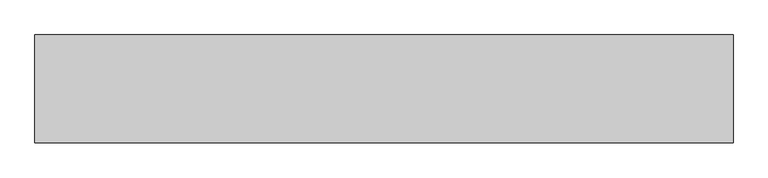
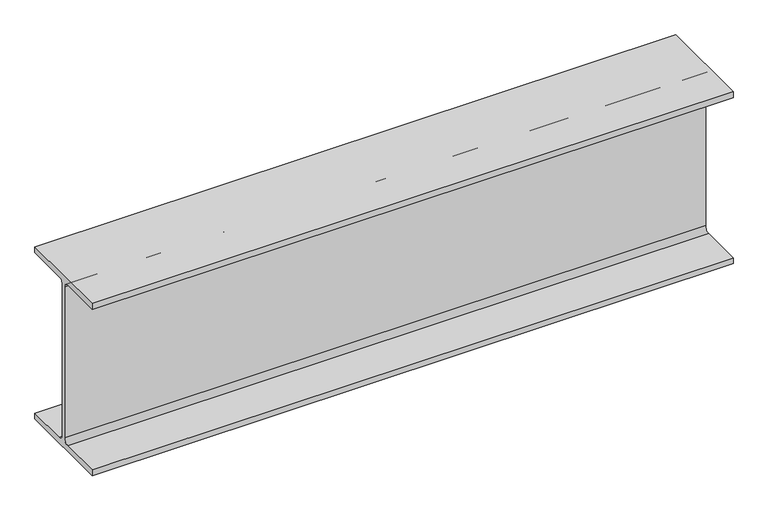
"""IFC4 building model written with IfcOpenShell, lengths in millimetres: beam geometry, Steel Beam_H-KSD3502 : H_SB_ASB_H-194x150x6x9."""

from ifc_helpers import new_model, si_unit, point, frame, frame_2d, origin, place, context, project, spatial, polyline, circle_curve, trimmed, segment, composite_curve, outline, extrude, source, transform, mapped, element, save


def beam_dbf2e1a8(model_context):
    return source(origin(), model_context, "Body", "SweptSolid", [
        extrude(outline(composite_curve([segment(polyline([(-82.5, -141.5), (-11.9, -141.5)]), True, "CONTINUOUS"), segment(trimmed(circle_curve(frame_2d((-11.9, -132.6)), 8.9), [point((-11.9, -141.5))], [point((-3.0, -132.6))], True, "CARTESIAN"), True, "CONTINUOUS"), segment(polyline([(-3.0, -132.6), (-3.0, 132.6)]), True, "CONTINUOUS"), segment(trimmed(circle_curve(frame_2d((-11.9, 132.6)), 8.9), [point((-3.0, 132.6))], [point((-11.9, 141.5))], True, "CARTESIAN"), True, "CONTINUOUS"), segment(polyline([(-11.9, 141.5), (-82.5, 141.5), (-82.5, 151.7), (82.5, 151.7), (82.5, 141.5), (11.9, 141.5)]), True, "CONTINUOUS"), segment(trimmed(circle_curve(frame_2d((11.9, 132.6)), 8.9), [point((11.9, 141.5))], [point((3.0, 132.6))], True, "CARTESIAN"), True, "CONTINUOUS"), segment(polyline([(3.0, 132.6), (3.0, -132.6)]), True, "CONTINUOUS"), segment(trimmed(circle_curve(frame_2d((11.9, -132.6)), 8.9), [point((3.0, -132.6))], [point((11.9, -141.5))], True, "CARTESIAN"), True, "CONTINUOUS"), segment(polyline([(11.9, -141.5), (82.5, -141.5), (82.5, -151.7), (-82.5, -151.7), (-82.5, -141.5)]), True, "CONTINUOUS")], self_intersect=False)), frame((-293.5180628, 0.0, 0.0), z_axis=(1.0, 0.0, 0.0), x_axis=(0.0, 1.0, 0.0)), (0.0, 0.0, 1.0), 1068.0320464),
    ])


if __name__ == "__main__":
    model = new_model("IFC4")
    model_context = context("Model", 3, world=origin())
    ifc_project = project(units=[si_unit("LENGTHUNIT", "METRE", prefix="MILLI")], contexts=[model_context])
    site = spatial("IfcSite", under=ifc_project)
    building = spatial("IfcBuilding", under=site)
    placement = place(None, origin())
    beam_shape = beam_dbf2e1a8(model_context)
    element("IfcBeam", 1, ObjectType="Steel Beam_H-KSD3502 : H_SB_ASB_H-194x150x6x9", at=placement, inside=building, context=model_context, shape_type="MappedRepresentation", body=[
        mapped(beam_shape, transform((0.0, 0.0, 0.0), x_axis=(1.0, 0.0, 0.0), y_axis=(0.0, 1.0, 0.0), z_axis=(0.0, 0.0, 1.0))),
    ])
    save(model, "model.ifc")

# Revit data of these elements
# Type "Steel Beam_H-KSD3502 : H_SB_ASB_H-194x150x6x9"
#   Width = 15.0 cm
#   Web Thickness = 0.6 cm
#   Web Fillet = 1.3 cm
#   Warping Constant = 43316.0 cm⁶
#   Torsional Moment of Inertia = 8.622 cm⁴
#   Torsional Modulus = 1.0 cm³
#   Section Area = 39.01 cm²
#   Plastic Modulus weak axis = 104.0 cm³
#   Plastic Modulus strong axis = 309.0 cm³
#   Perimeter = 0.95 m²/m
#   Nominal Weight = 30.60 kgf/m
#   Moment of Inertia weak axis = 507.00 cm⁴
#   Moment of Inertia strong axis = 2690.00 cm⁴
#   Height = 19.4 cm
#   Flange Thickness = 0.9 cm
#   Elastic Modulus weak axis = 67.6 cm³
#   Elastic Modulus strong axis = 277.0 cm³
#   Centroid Vertical = 9.7 cm
#   Centroid Horizontal = 7.5 cm
#   Length [instance default] = 1.5240 m
#   Structural Material [instance default] = Steel, 45-345
#   Assembly Code = ""
# Element 1 (IfcBeam, "Steel Beam_H-KSD3502 : H_SB_ASB_H-194x150x6x9")
#   Structural Material = none
# Materials
#   "Steel, 45-345": class "Metal", colour RGB 189 187 185, transparency 0, Description = "Steel 345 MPa", Cost = 0
